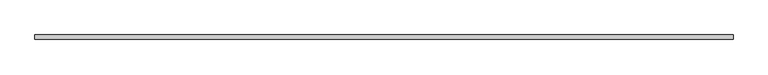
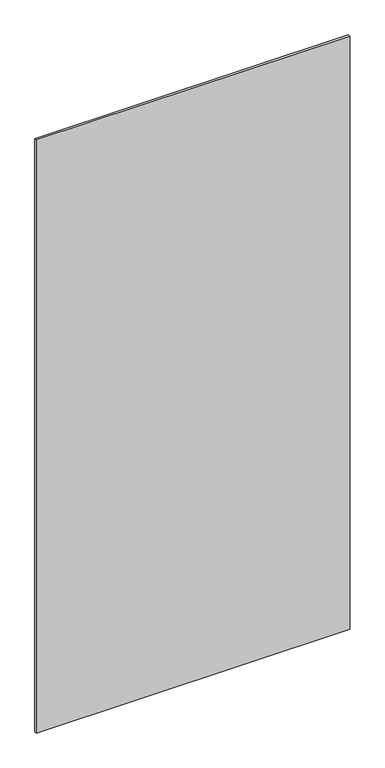
"""IFC4 building model written with IfcOpenShell, lengths in millimetres: proxy geometry, Panel:Panel:300402:Panel:300402 : Panel:Panel:300402:300124:Panel:300402:Panel:300402 : Panel:Panel:300402:300124 : Panel:Panel:300402:Panel:300402 : Panel:Panel:300402:300124:3 : Panel:Panel:300402:Panel:300402 : Panel:Panel:300402:300124:Panel:300402:Panel:300402 : Panel:Panel:300402:300124 : Panel:Panel:300402:Panel:300402 : Panel:Panel:300402:300124:300083."""

from ifc_helpers import new_model, si_unit, frame, origin, place, context, project, spatial, polyline, outline, extrude, source, transform, mapped, element, save


def generic_models_84dc123e(model_context):
    return source(origin(), model_context, "Body", "SweptSolid", [
        extrude(outline(polyline([(570452.6367239, -579076.8913841), (571671.8367239, -579076.8913841), (571671.8367239, -579084.8288841), (570452.6367239, -579084.8288841), (570452.6367239, -579076.8913841)])), frame((0.0, 0.0, 2470.15), z_axis=(0.0, 0.0, 1.0), x_axis=(1.0, 0.0, 0.0)), (0.0, 0.0, 1.0), 2438.4),
    ])


if __name__ == "__main__":
    model = new_model("IFC4")
    model_context = context("Model", 3, world=origin())
    ifc_project = project(units=[si_unit("LENGTHUNIT", "METRE", prefix="MILLI")], contexts=[model_context])
    site = spatial("IfcSite", under=ifc_project)
    building = spatial("IfcBuilding", under=site)
    placement = place(None, origin())
    generic_models_shape = generic_models_84dc123e(model_context)
    element("IfcBuildingElementProxy", 1, Name="Panel:Panel:300402:Panel:300402 : Panel:Panel:300402:300124:Panel:300402:Panel:300402 : Panel:Panel:300402:300124 : Panel:Panel:300402:Panel:300402 : Panel:Panel:300402:300124:3 : Panel:Panel:300402:Panel:300402 : Panel:Panel:300402:300124:Panel:300402:Panel:300402 : Panel:Panel:300402:300124 : Panel:Panel:300402:Panel:300402 : Panel:Panel:300402:300124:300083", ObjectType="Panel:Panel:300402:Panel:300402 : Panel:Panel:300402:300124:Panel:300402:Panel:300402 : Panel:Panel:300402:300124 : Panel:Panel:300402:Panel:300402 : Panel:Panel:300402:300124:3 : Panel:Panel:300402:Panel:300402 : Panel:Panel:300402:300124:Panel:300402:Panel:300402 : Panel:Panel:300402:300124 : Panel:Panel:300402:Panel:300402 : Panel:Panel:300402:300124:300083", at=placement, inside=building, context=model_context, shape_type="MappedRepresentation", body=[
        mapped(generic_models_shape, transform((0.0, 0.0, 0.0), x_axis=(1.0, 0.0, 0.0), y_axis=(0.0, 1.0, 0.0), z_axis=(0.0, 0.0, 1.0))),
    ])
    save(model, "model.ifc")

# Revit data of these elements
# Type "Panel:Panel:300402:Panel:300402 : Panel:Panel:300402:300124:Panel:300402:Panel:300402 : Panel:Panel:300402:300124 : Panel:Panel:300402:Panel:300402 : Panel:Panel:300402:300124:3 : Panel:Panel:300402:Panel:300402 : Panel:Panel:300402:300124:Panel:300402:Panel:300402 : Panel:Panel:300402:300124 : Panel:Panel:300402:Panel:300402 : Panel:Panel:300402:300124:300083"
#   NameOverride = "Panel:Panel:300402:Panel:300402 : Panel:Panel:300402:300124:Panel:300402:Panel:300402 : Panel:Panel:300402:300124 : Panel:Panel:300402:Panel:300402 : Panel:Panel:300402:300124:300083"
#   ObjectTypeOverride = "Panel:300402:Panel:300402 : Panel:Panel:300402:300124 : Panel:Panel:300402:Panel:300402 : Panel:Panel:300402:300124"
#   Reference = "Panel"
#   Tag = "300083"
# Element 1 (IfcBuildingElementProxy, "Panel:Panel:300402:Panel:300402 : Panel:Panel:300402:300124:Panel:300402:Panel:300402 : Panel:Panel:300402:300124 : Panel:Panel:300402:Panel:300402 : Panel:Panel:300402:300124:3 : Panel:Panel:300402:Panel:300402 : Panel:Panel:300402:300124:Panel:300402:Panel:300402 : Panel:Panel:300402:300124 : Panel:Panel:300402:Panel:300402 : Panel:Panel:300402:300124:300083")
#   Materials on its faces: "5/16\" PHENOLIC RESIN PANELS (CLASS A FLAME SPREAD) - EXPOSED FASTENERS"
# Materials
#   "5/16\" PHENOLIC RESIN PANELS (CLASS A FLAME SPREAD) - EXPOSED FASTENERS": class "Unassigned", colour RGB 64 64 64, transparency 0, Keynote = "M07420000.01", Cost = 0
